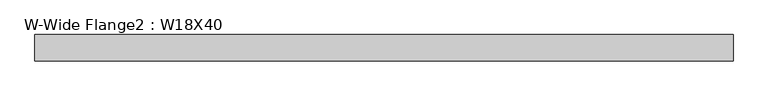
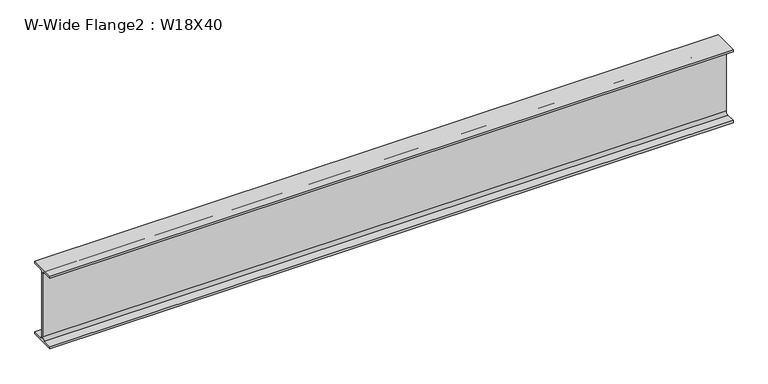
"""IFC4 building model written with IfcOpenShell, lengths in millimetres: beam geometry, W-Wide Flange2 : W18X40."""

from ifc_helpers import new_model, si_unit, point, frame, frame_2d, origin, place, context, project, spatial, polyline, circle_curve, trimmed, segment, composite_curve, outline, extrude, source, transform, mapped, element, save


def w_wide_flange2_w18x40_35389f5a(model_context):
    return source(origin(), model_context, "Body", "SweptSolid", [
        extrude(outline(composite_curve([segment(polyline([(76.454, -213.995), (76.454, -227.33), (-76.454, -227.33), (-76.454, -213.995), (-20.828, -213.995)]), True, "CONTINUOUS"), segment(trimmed(circle_curve(frame_2d((-20.828, -197.1675)), 16.8275), [point((-20.828, -213.995))], [point((-4.0005, -197.1675))], True, "CARTESIAN"), True, "CONTINUOUS"), segment(polyline([(-4.0005, -197.1675), (-4.0005, 197.1675)]), True, "CONTINUOUS"), segment(trimmed(circle_curve(frame_2d((-20.828, 197.1675)), 16.8275), [point((-4.0005, 197.1675))], [point((-20.828, 213.995))], True, "CARTESIAN"), True, "CONTINUOUS"), segment(polyline([(-20.828, 213.995), (-76.454, 213.995), (-76.454, 227.33), (76.454, 227.33), (76.454, 213.995), (20.828, 213.995)]), True, "CONTINUOUS"), segment(trimmed(circle_curve(frame_2d((20.828, 197.1675)), 16.8275), [point((20.828, 213.995))], [point((4.0005, 197.1675))], True, "CARTESIAN"), True, "CONTINUOUS"), segment(polyline([(4.0005, 197.1675), (4.0005, -197.1675)]), True, "CONTINUOUS"), segment(trimmed(circle_curve(frame_2d((20.828, -197.1675)), 16.8275), [point((4.0005, -197.1675))], [point((20.828, -213.995))], True, "CARTESIAN"), True, "CONTINUOUS"), segment(polyline([(20.828, -213.995), (76.454, -213.995)]), True, "CONTINUOUS")], self_intersect=False)), frame((-2017.7125, 0.0, 0.0), z_axis=(1.0, 0.0, 0.0), x_axis=(0.0, 1.0, 0.0)), (0.0, 0.0, 1.0), 4035.425),
    ])


if __name__ == "__main__":
    model = new_model("IFC4")
    model_context = context("Model", 3, world=origin())
    ifc_project = project(units=[si_unit("LENGTHUNIT", "METRE", prefix="MILLI")], contexts=[model_context])
    site = spatial("IfcSite", under=ifc_project)
    building = spatial("IfcBuilding", under=site)
    placement = place(None, origin())
    w_wide_flange2_w18x40_shape = w_wide_flange2_w18x40_35389f5a(model_context)
    element("IfcBeam", 1, ObjectType="W-Wide Flange2 : W18X40", at=placement, inside=building, context=model_context, shape_type="MappedRepresentation", body=[
        mapped(w_wide_flange2_w18x40_shape, transform((0.0, 0.0, 0.0), x_axis=(1.0, 0.0, 0.0), y_axis=(0.0, 1.0, 0.0), z_axis=(0.0, 0.0, 1.0))),
    ])
    save(model, "model.ifc")

# Revit data of these elements
# Type "W-Wide Flange2 : W18X40"
#   Assembly Code = "B10"
#   W = 40
#   Length [instance default] = 5' - 0"
#   bf = 0' - 6.02"
#   d = 1' - 5.9"
#   k = 0' - 1 3/16"
#   k2 = 0' - 0.6625"
#   tf = 0' - 0.525"
#   tw = 0' - 0.315"
#   A = 0.0819444 SF
#   Structural Material [instance default] = Steel ASTM A992
# Element 1 (IfcBeam, "W-Wide Flange2 : W18X40")
#   Materials on its faces: "Steel ASTM A992"
# Materials
#   "Steel ASTM A992": class "Metal", colour RGB 199 199 199, transparency 0, Description = "Structural steel 50ksi", Cost = 0
